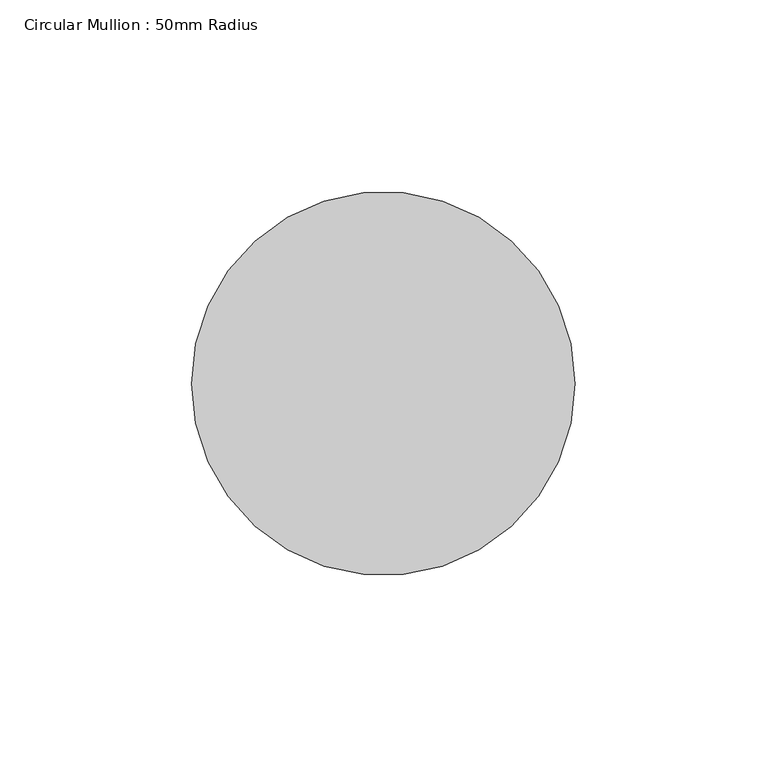
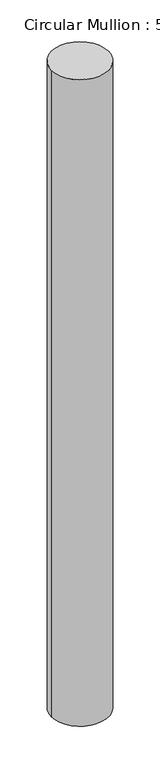
"""IFC4 building model written with IfcOpenShell, lengths in millimetres: member geometry, Circular Mullion : 50mm Radius."""

from ifc_helpers import new_model, si_unit, point, frame, origin, origin_2d, place, context, project, spatial, circle_curve, trimmed, segment, composite_curve, outline, extrude, source, transform, mapped, element, save


def circular_mullion_50mm_radius_9b2805d5(model_context):
    return source(origin(), model_context, "Body", "SweptSolid", [
        extrude(outline(composite_curve([segment(trimmed(circle_curve(origin_2d(), 50.0), [point((50.0, 0.0))], [point((-50.0, 0.0))], False, "CARTESIAN"), True, "CONTINUOUS"), segment(trimmed(circle_curve(origin_2d(), 50.0), [point((-50.0, 0.0))], [point((50.0, 0.0))], False, "CARTESIAN"), True, "CONTINUOUS")], self_intersect=False)), frame((0.0, 0.0, -1196.7650446), z_axis=(0.0, 0.0, 1.0), x_axis=(1.0, 0.0, 0.0)), (0.0, 0.0, 1.0), 1196.7650446),
    ])


if __name__ == "__main__":
    model = new_model("IFC4")
    model_context = context("Model", 3, world=origin())
    ifc_project = project(units=[si_unit("LENGTHUNIT", "METRE", prefix="MILLI")], contexts=[model_context])
    site = spatial("IfcSite", under=ifc_project)
    building = spatial("IfcBuilding", under=site)
    placement = place(None, origin())
    circular_mullion_50mm_radius_shape = circular_mullion_50mm_radius_9b2805d5(model_context)
    element("IfcMember", 1, ObjectType="Circular Mullion : 50mm Radius", at=placement, inside=building, context=model_context, shape_type="MappedRepresentation", body=[
        mapped(circular_mullion_50mm_radius_shape, transform((0.0, 0.0, 0.0), x_axis=(1.0, 0.0, 0.0), y_axis=(0.0, 1.0, 0.0), z_axis=(0.0, 0.0, 1.0))),
    ])
    save(model, "model.ifc")

# Revit data of these elements
# Type "Circular Mullion : 50mm Radius"
#   built-in parameter 1007350 = 0.164042 (stored number, unit not read)
# Element 1 (IfcMember, "Circular Mullion : 50mm Radius")
#   Materials on its faces: "Aluminium"
# Materials
#   "Aluminium": class "Metal", colour RGB 247 247 247, transparency 0, Description = "Aluminium 6061", Cost = 0
